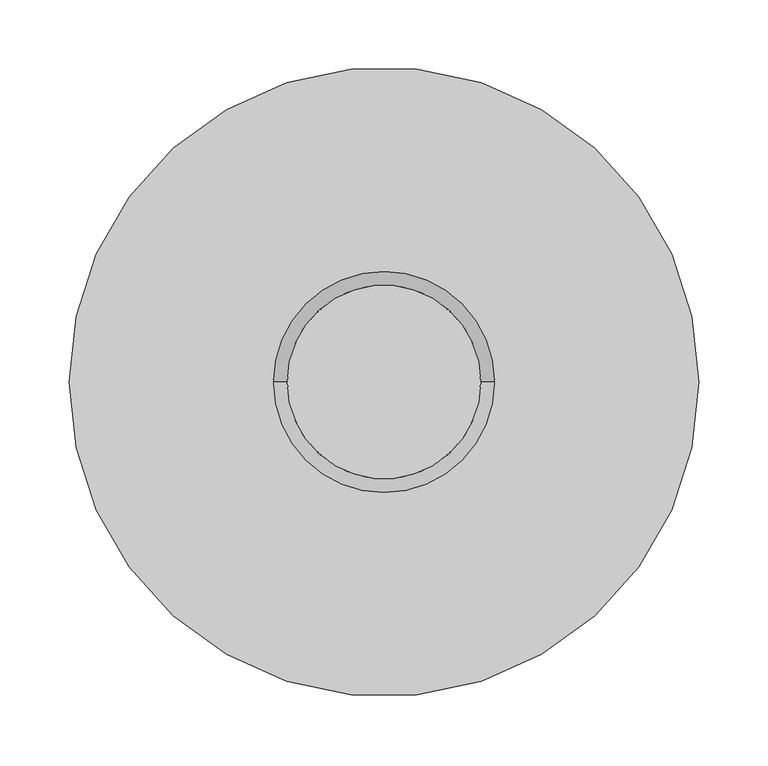
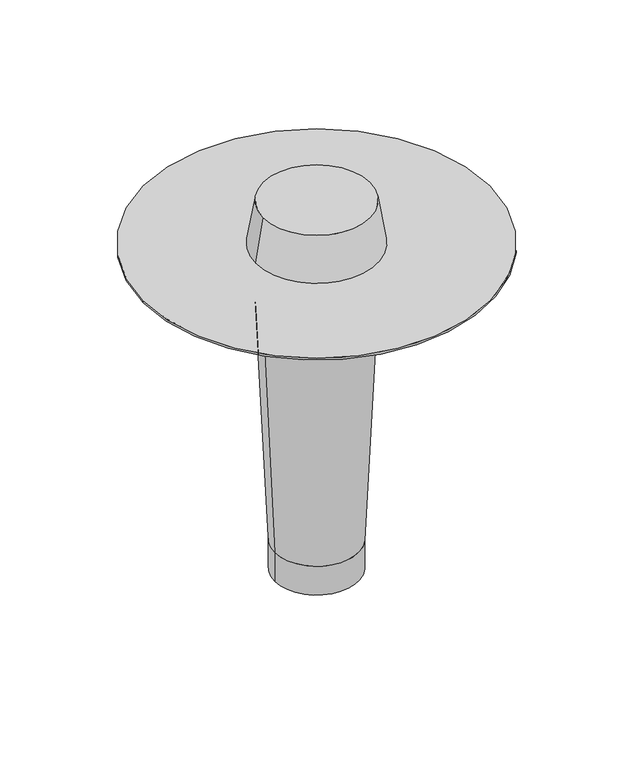
"""IFC4 building model written with IfcOpenShell, lengths in millimetres: proxy geometry, TN_Воронка ТехноНИКОЛЬ ВБ : Воронка ТехноНИКОЛЬ ВБ, 110х450."""

from ifc_helpers import new_model, si_unit, point, frame, origin, origin_2d, place, context, project, spatial, polyline, circle_curve, trimmed, segment, composite_curve, outline, extrude, source, transform, mapped, element, save
from ifc_brep_helpers import plane_surface, revolved_surface, advanced_brep


def specialty_equipment_32c1bbf0(model_context):
    return source(origin(), model_context, "Body", "SolidModel", [
        advanced_brep(
        [(70.0, 0.0, -85.0), (-70.0, 0.0, -85.0), (55.0, 0.0, -410.0), (-55.0, 0.0, -410.0)],
        [
            (0, 1, circle_curve(frame((0.0, 0.0, -85.0), z_axis=(0.0, 0.0, 1.0), x_axis=(1.0, 0.0, 0.0)), 70.0)),
            (1, 0, circle_curve(frame((0.0, 0.0, -85.0), z_axis=(0.0, 0.0, 1.0), x_axis=(-1.0, 0.0, 0.0)), 70.0)),
            (2, 3, circle_curve(frame((0.0, 0.0, -410.0), z_axis=(0.0, 0.0, -1.0), x_axis=(-1.0, 0.0, 0.0)), 55.0)),
            (3, 2, circle_curve(frame((0.0, 0.0, -410.0), z_axis=(0.0, 0.0, -1.0), x_axis=(1.0, 0.0, 0.0)), 55.0)),
            (3, 1),
            (0, 2),
        ],
        [
            plane_surface(frame((0.0, 0.0, -85.0), z_axis=(0.0, 0.0, 1.0), x_axis=(0.0, 1.0, 0.0))),
            plane_surface(frame((0.0, 0.0, -410.0), z_axis=(0.0, 0.0, -1.0), x_axis=(0.0, 1.0, 0.0))),
            revolved_surface(polyline([(-55.00000000032967, 0.0, -410.0), (-70.0, 0.0, -85.0)]), (0.0, 0.0, -1601.6666667), (0.0, 0.0, 1.0)),
            revolved_surface(polyline([(55.00000000032967, 0.0, -410.0), (70.0, 0.0, -85.0)]), (0.0, 0.0, -1601.6666667), (0.0, 0.0, 1.0)),
        ],
        [
            (0, [[1, 2]]),
            (1, [[3, 4]]),
            (2, [[-4, 5, -1, 6]]),
            (3, [[-3, -6, -2, -5]]),
        ],
    ),
        extrude(outline(composite_curve([segment(trimmed(circle_curve(origin_2d(), 70.0), [point((-70.0, 0.0))], [point((70.0, 0.0))], False, "CARTESIAN"), True, "CONTINUOUS"), segment(trimmed(circle_curve(origin_2d(), 70.0), [point((70.0, 0.0))], [point((-70.0, 0.0))], False, "CARTESIAN"), True, "CONTINUOUS")], self_intersect=False)), frame((0.0, 0.0, -85.0), z_axis=(0.0, 0.0, 1.0), x_axis=(1.0, 0.0, 0.0)), (0.0, 0.0, 1.0), 82.0),
        extrude(outline(composite_curve([segment(trimmed(circle_curve(origin_2d(), 55.0), [point((55.0, 0.0))], [point((-55.0, 0.0))], False, "CARTESIAN"), True, "CONTINUOUS"), segment(trimmed(circle_curve(origin_2d(), 55.0), [point((-55.0, 0.0))], [point((55.0, 0.0))], False, "CARTESIAN"), True, "CONTINUOUS")], self_intersect=False)), frame((0.0, 0.0, -450.0), z_axis=(0.0, 0.0, 1.0), x_axis=(1.0, 0.0, 0.0)), (0.0, 0.0, 1.0), 40.0),
        extrude(outline(composite_curve([segment(trimmed(circle_curve(origin_2d(), 227.5), [point((-227.5, 0.0))], [point((227.5, 0.0))], False, "CARTESIAN"), True, "CONTINUOUS"), segment(trimmed(circle_curve(origin_2d(), 227.5), [point((227.5, 0.0))], [point((-227.5, 0.0))], False, "CARTESIAN"), True, "CONTINUOUS")], self_intersect=False)), frame((0.0, 0.0, -3.0), z_axis=(0.0, 0.0, 1.0), x_axis=(1.0, 0.0, 0.0)), (0.0, 0.0, 1.0), 3.0),
        advanced_brep(
        [(-70.0, 0.0, 60.0), (70.0, 0.0, 60.0), (-80.0, 0.0, 0.0), (80.0, 0.0, 0.0)],
        [
            (0, 1, circle_curve(frame((0.0, 0.0, 60.0), z_axis=(0.0, 0.0, 1.0), x_axis=(-1.0, 0.0, 0.0)), 70.0)),
            (1, 0, circle_curve(frame((0.0, 0.0, 60.0), z_axis=(0.0, 0.0, 1.0), x_axis=(1.0, 0.0, 0.0)), 70.0)),
            (2, 3, circle_curve(frame((0.0, 0.0, 0.0), z_axis=(0.0, 0.0, -1.0), x_axis=(1.0, 0.0, 0.0)), 80.0)),
            (3, 2, circle_curve(frame((0.0, 0.0, 0.0), z_axis=(0.0, 0.0, -1.0), x_axis=(-1.0, 0.0, 0.0)), 80.0)),
            (3, 1),
            (0, 2),
        ],
        [
            plane_surface(frame((0.0, 0.0, 60.0), z_axis=(0.0, 0.0, 1.0), x_axis=(0.0, -1.0, 0.0))),
            plane_surface(frame((0.0, 0.0, 0.0), z_axis=(0.0, 0.0, -1.0), x_axis=(0.0, -1.0, 0.0))),
            revolved_surface(polyline([(-70.0, 0.0, 60.0), (-80.0, 0.0, 0.0)]), (0.0, 0.0, 480.0), (0.0, 0.0, -1.0)),
            revolved_surface(polyline([(70.0, 0.0, 60.0), (80.0, 0.0, 0.0)]), (0.0, 0.0, 480.0), (0.0, 0.0, -1.0)),
        ],
        [
            (0, [[1, 2]]),
            (1, [[3, 4]]),
            (2, [[-4, 5, -1, 6]]),
            (3, [[-3, -6, -2, -5]]),
        ],
    ),
    ])


if __name__ == "__main__":
    model = new_model("IFC4")
    model_context = context("Model", 3, world=origin())
    ifc_project = project(units=[si_unit("LENGTHUNIT", "METRE", prefix="MILLI")], contexts=[model_context])
    site = spatial("IfcSite", under=ifc_project)
    building = spatial("IfcBuilding", under=site)
    placement = place(None, origin())
    specialty_equipment_shape = specialty_equipment_32c1bbf0(model_context)
    element("IfcBuildingElementProxy", 1, Name="TN_Воронка ТехноНИКОЛЬ ВБ : Воронка ТехноНИКОЛЬ ВБ, 110х450", ObjectType="TN_Воронка ТехноНИКОЛЬ ВБ : Воронка ТехноНИКОЛЬ ВБ, 110х450", at=placement, inside=building, context=model_context, shape_type="MappedRepresentation", body=[
        mapped(specialty_equipment_shape, transform((0.0, 0.0, 0.0), x_axis=(1.0, 0.0, 0.0), y_axis=(0.0, 1.0, 0.0), z_axis=(0.0, 0.0, 1.0))),
    ])
    save(model, "model.ifc")

# Revit data of these elements
# Type "TN_Воронка ТехноНИКОЛЬ ВБ : Воронка ТехноНИКОЛЬ ВБ, 110х450"
#   ADSK_Группирование = "Комплектующие и воронки"
#   Description = "Воронка ВБ используется при ремонте и строительстве зданий и сооружений и предназначена для\nудаления дождевой воды с плоских кровель. Применяется в кровлях из битумных и битумно-полимерных\nрулонных и мастичных материалов с внутренним водостоком. Рекомендуется устанавливать одну\nворонку примерно на каждые 250 м2 кровли, но требуется не менее двух водоотводящих систем на\nкровлю ограниченную парапетами. Пропуская способность 7,8 л/сек."
#   Manufacturer = "ТехноНИКОЛЬ"
#   URL = "http://nav.tn.ru/upload/iblock/67f/67f1681bb0d078f2e8af03b9528f2af6.pdf"
#   ADSK_Примечание = ""
#   ADSK_Обозначение = "ТехноНИКОЛЬ"
#   ADSK_Наименование = "Воронка ТехноНИКОЛЬ ВБ, 110х450"
#   ADSK_Марка = ""
#   ADSK_Код изделия = "460062"
#   ADSK_Завод-изготовитель = "ТехноНИКОЛЬ"
#   ADSK_Единица измерения = "шт."
#   ADSK_Группирование = "Комплектующие и воронки"
#   ADSK_URL страницы изделия = "https://shop.tn.ru/voronka-tehnonikol-vb-110h450-mm"
#   ADSK_URL документации изделия = "https://nav.tn.ru/upload/iblock/b23/Tekhlist-7.17_Voronka_BV_110_-30.01.2014.pdf"
#   Диаметр фланца = 455 mm
#   Высота воронки = 450 mm
#   ADSK_Масса = 1.65
#   ADSK_Количество = 1
#   Материал = TN_ПВХ_Черный
#   Default Elevation = 0
# Element 1 (IfcBuildingElementProxy, "TN_Воронка ТехноНИКОЛЬ ВБ : Воронка ТехноНИКОЛЬ ВБ, 110х450")
#   Materials on its faces: "TN_ПВХ_Черный"
# Materials
#   "TN_ПВХ_Черный": class "Типовые", colour RGB 48 48 48, transparency 0, Cost = 0
